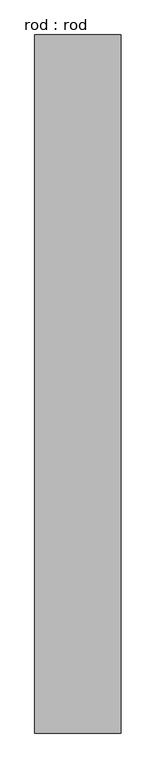
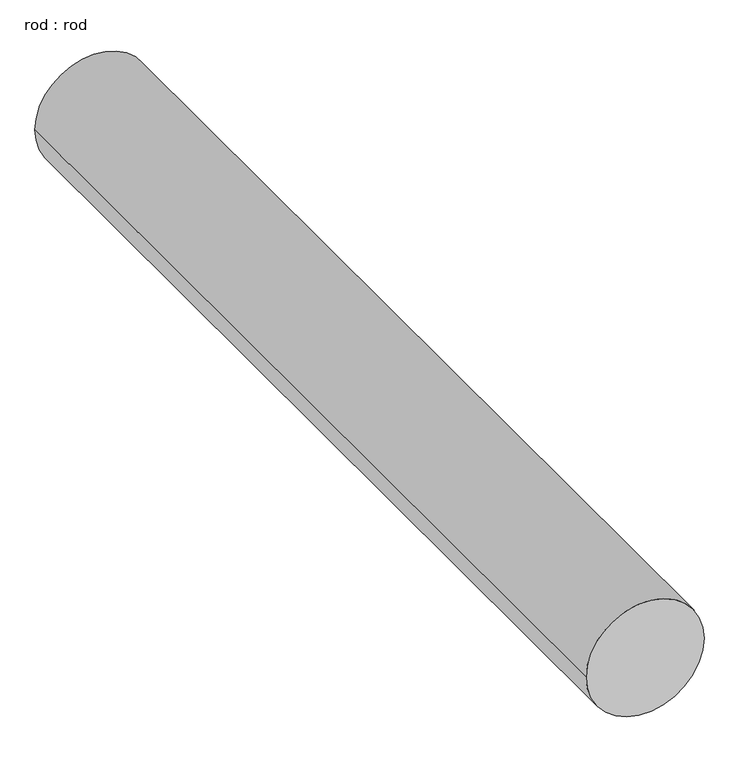
"""IFC4 building model written with IfcOpenShell, lengths in millimetres: proxy geometry, rod : rod."""

from ifc_helpers import new_model, si_unit, point, frame, frame_2d, origin, place, context, project, spatial, circle_curve, trimmed, segment, composite_curve, outline, extrude, source, transform, mapped, element, save


def rod_rod_b34b8398(model_context):
    return source(origin(), model_context, "Body", "SweptSolid", [
        extrude(outline(composite_curve([segment(trimmed(circle_curve(frame_2d((0.0108462, 0.0)), 200.0), [point((0.0108462, 200.0))], [point((0.0108462, -200.0))], False, "CARTESIAN"), True, "CONTINUOUS"), segment(trimmed(circle_curve(frame_2d((0.0108462, 0.0)), 200.0), [point((0.0108462, -200.0))], [point((0.0108462, 200.0))], False, "CARTESIAN"), True, "CONTINUOUS")], self_intersect=False)), frame((0.0, 2474.8714725, 0.0), z_axis=(0.0, 1.0, 0.0), x_axis=(0.0, 0.0, 1.0)), (0.0, 0.0, 1.0), 3235.7142857),
    ])


if __name__ == "__main__":
    model = new_model("IFC4")
    model_context = context("Model", 3, world=origin())
    ifc_project = project(units=[si_unit("LENGTHUNIT", "METRE", prefix="MILLI")], contexts=[model_context])
    site = spatial("IfcSite", under=ifc_project)
    building = spatial("IfcBuilding", under=site)
    placement = place(None, origin())
    rod_rod_shape = rod_rod_b34b8398(model_context)
    element("IfcBuildingElementProxy", 1, Name="rod : rod", ObjectType="rod : rod", at=placement, inside=building, context=model_context, shape_type="MappedRepresentation", body=[
        mapped(rod_rod_shape, transform((0.0, 0.0, 0.0), x_axis=(1.0, 0.0, 0.0), y_axis=(0.0, 1.0, 0.0), z_axis=(0.0, 0.0, 1.0))),
    ])
    save(model, "model.ifc")

# Revit data of these elements
# Type "rod : rod"
#   Default Elevation = 0
